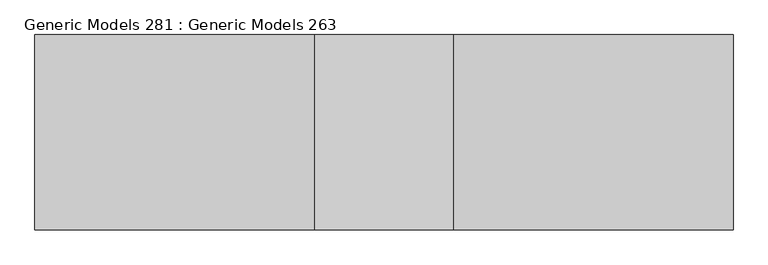
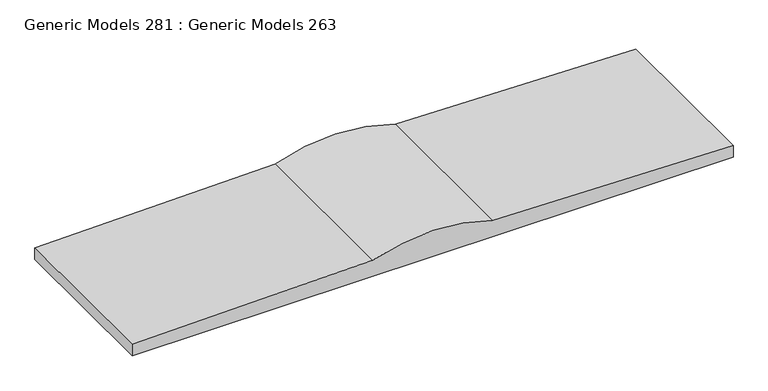
"""IFC4 building model written with IfcOpenShell, lengths in millimetres: proxy geometry, Generic Models 281 : Generic Models 263."""

from ifc_helpers import new_model, si_unit, point, frame, frame_2d, origin, place, context, project, spatial, polyline, circle_curve, trimmed, segment, composite_curve, outline, extrude, source, transform, mapped, element, save


def generic_models_281_generic_models_263_cbb34a41(model_context):
    return source(origin(), model_context, "Body", "SweptSolid", [
        extrude(outline(composite_curve([segment(polyline([(0.0, 64122.5797726), (-304.9836851, 64122.5797726)]), True, "CONTINUOUS"), segment(trimmed(circle_curve(frame_2d((-219607.3320282, 71742.5797726)), 219434.6927648), [point((-304.9836851, 64122.5797726))], [point((-304.9836851, 79362.5797726))], True, "CARTESIAN"), True, "CONTINUOUS"), segment(polyline([(-304.9836851, 79362.5797726), (0.0, 79362.5797726)]), True, "CONTINUOUS"), segment(trimmed(circle_curve(frame_2d((-219607.3320282, 71742.5797726)), 219739.4927648), [point((0.0, 79362.5797726))], [point((126.8758334, 73266.5797726))], False, "CARTESIAN"), True, "CONTINUOUS"), segment(trimmed(circle_curve(frame_2d((-4163.1944851, 71742.5797726)), 4552.7221898), [point((126.8758334, 73266.5797726))], [point((126.8758334, 70218.5797726))], False, "CARTESIAN"), True, "CONTINUOUS"), segment(trimmed(circle_curve(frame_2d((-219607.3320282, 71742.5797726)), 219739.4927648), [point((126.8758334, 70218.5797726))], [point((0.0, 64122.5797726))], False, "CARTESIAN"), True, "CONTINUOUS")], self_intersect=False)), frame((0.0, -1618.4486541, 0.0), z_axis=(0.0, 1.0, 0.0), x_axis=(0.0, 0.0, 1.0)), (0.0, 0.0, 1.0), 4267.2),
    ])


if __name__ == "__main__":
    model = new_model("IFC4")
    model_context = context("Model", 3, world=origin())
    ifc_project = project(units=[si_unit("LENGTHUNIT", "METRE", prefix="MILLI")], contexts=[model_context])
    site = spatial("IfcSite", under=ifc_project)
    building = spatial("IfcBuilding", under=site)
    placement = place(None, origin())
    generic_models_281_generic_models_263_shape = generic_models_281_generic_models_263_cbb34a41(model_context)
    element("IfcBuildingElementProxy", 1, Name="Generic Models 281 : Generic Models 263", ObjectType="Generic Models 281 : Generic Models 263", at=placement, inside=building, context=model_context, shape_type="MappedRepresentation", body=[
        mapped(generic_models_281_generic_models_263_shape, transform((0.0, 0.0, 0.0), x_axis=(1.0, 0.0, 0.0), y_axis=(0.0, 1.0, 0.0), z_axis=(0.0, 0.0, 1.0))),
    ])
    save(model, "model.ifc")

# Revit data of these elements
# Element 1 (IfcBuildingElementProxy, "Generic Models 281 : Generic Models 263")
#   Materials on its faces: "3\" TO 6\" WASHED OR CLEAR STONE"
# Materials
#   "3\" TO 6\" WASHED OR CLEAR STONE": class "Miscellaneous", colour RGB 210 210 210, transparency 0, Cost = 0
